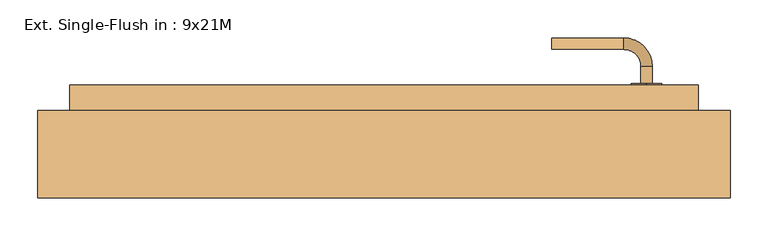
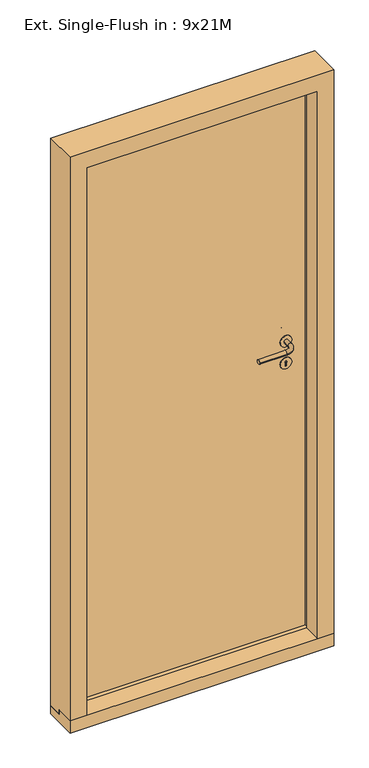
"""IFC4 building model written with IfcOpenShell, lengths in millimetres: door geometry, Ext. Single-Flush in : 9x21M."""

from ifc_helpers import new_model, si_unit, point, frame, frame_2d, origin, place, context, project, spatial, polyline, circle_curve, ellipse_curve, trimmed, segment, composite_curve, outline, extrude, faceted_brep, source, transform, mapped, element, save
from ifc_brep_helpers import plane_surface, cylinder_surface, revolved_surface, advanced_brep


def ext_single_flush_in_9x21m_f1e34a21(model_context):
    return source(origin(), model_context, "Body", "SolidModel", [
        extrude(outline(composite_curve([segment(trimmed(circle_curve(frame_2d((1090.0, 346.0)), 20.0), [point((1070.0, 346.0))], [point((1110.0, 346.0))], False, "CARTESIAN"), True, "CONTINUOUS"), segment(trimmed(circle_curve(frame_2d((1090.0, 346.0)), 20.0), [point((1110.0, 346.0))], [point((1070.0, 346.0))], False, "CARTESIAN"), True, "CONTINUOUS")], self_intersect=False)), frame((0.0, -35.0, 0.0), z_axis=(0.0, 1.0, 0.0), x_axis=(0.0, 0.0, 1.0)), (0.0, 0.0, 1.0), 2.0),
        advanced_brep(
        [(353.5, -33.0, 1090.0), (338.5, -33.0, 1090.0), (338.5, -10.5, 1090.0), (353.5, -10.5, 1090.0), (316.0, 12.0, 1090.0), (316.0, 27.0, 1090.0), (221.0, 12.0, 1090.0), (221.0, 27.0, 1090.0)],
        [
            (0, 1, circle_curve(frame((346.0, -33.0, 1090.0), z_axis=(0.0, -1.0, 0.0), x_axis=(-1.0, 0.0, 0.0)), 7.5)),
            (1, 0, circle_curve(frame((346.0, -33.0, 1090.0), z_axis=(0.0, -1.0, 0.0), x_axis=(-1.0, 0.0, 0.0)), 7.5)),
            (1, 2),
            (2, 3, circle_curve(frame((346.0, -10.5, 1090.0), z_axis=(0.0, -1.0, 0.0), x_axis=(-1.0, 0.0, 0.0)), 7.5)),
            (3, 0),
            (3, 2, circle_curve(frame((346.0, -10.5, 1090.0), z_axis=(0.0, -1.0, 0.0), x_axis=(-1.0, 0.0, 0.0)), 7.5)),
            (4, 5, circle_curve(frame((316.0, 19.5, 1090.0), z_axis=(1.0, 0.0, 0.0), x_axis=(0.0, -1.0, 0.0)), 7.5)),
            (5, 3, circle_curve(frame((316.0, -10.5, 1090.0), z_axis=(0.0, 0.0, -1.0), x_axis=(1.0, 0.0, 0.0)), 37.5)),
            (2, 4, circle_curve(frame((316.0, -10.5, 1090.0), z_axis=(0.0, 0.0, 1.0), x_axis=(1.0, 0.0, 0.0)), 22.5)),
            (5, 4, circle_curve(frame((316.0, 19.5, 1090.0), z_axis=(1.0, 0.0, 0.0), x_axis=(0.0, -1.0, 0.0)), 7.5)),
            (4, 6),
            (6, 7, circle_curve(frame((221.0, 19.5, 1090.0), z_axis=(1.0, 0.0, 0.0), x_axis=(0.0, -1.0, 0.0)), 7.5)),
            (7, 5),
            (7, 6, circle_curve(frame((221.0, 19.5, 1090.0), z_axis=(1.0, 0.0, 0.0), x_axis=(0.0, -1.0, 0.0)), 7.5)),
        ],
        [
            plane_surface(frame((346.0, -33.0, 1090.0), z_axis=(0.0, -1.0, 0.0), x_axis=(0.0, 0.0, -1.0))),
            cylinder_surface(frame((346.0, -33.0, 1090.0), z_axis=(0.0, -1.0, 0.0), x_axis=(-1.0, 0.0, 0.0)), 7.5),
            revolved_surface(trimmed(ellipse_curve(frame((346.0, -10.5, 1090.0), z_axis=(0.0, 1.0, 0.0), x_axis=(-1.0, 0.0, 0.0)), 7.5, 7.5), [point((353.5, -10.5, 1090.0))], [point((338.5, -10.5, 1090.0))], True, "CARTESIAN"), (316.0, -10.5, 1090.0), (0.0, 0.0, -1.0)),
            revolved_surface(trimmed(ellipse_curve(frame((346.0, -10.5, 1090.0), z_axis=(0.0, 1.0, 0.0), x_axis=(-1.0, 0.0, 0.0)), 7.5, 7.5), [point((338.5, -10.5, 1090.0))], [point((353.5, -10.5, 1090.0))], True, "CARTESIAN"), (316.0, -10.5, 1090.0), (0.0, 0.0, -1.0)),
            cylinder_surface(frame((316.0, 19.5, 1090.0), z_axis=(1.0, 0.0, 0.0), x_axis=(0.0, -1.0, 0.0)), 7.5),
            plane_surface(frame((221.0, 19.5, 1090.0), z_axis=(-1.0, 0.0, 0.0), x_axis=(0.0, 0.0, -1.0))),
        ],
        [
            (0, [[1, 2]]),
            (1, [[3, 4, 5, -2]]),
            (1, [[-5, 6, -3, -1]]),
            (2, [[7, 8, -4, 9]]),
            (3, [[10, -9, -6, -8]]),
            (4, [[11, 12, 13, -7]]),
            (4, [[-13, 14, -11, -10]]),
            (5, [[-12, -14]]),
        ],
    ),
        extrude(outline(composite_curve([segment(trimmed(circle_curve(frame_2d((1010.0, 346.0)), 20.0), [point((990.0, 346.0))], [point((1030.0, 346.0))], False, "CARTESIAN"), True, "CONTINUOUS"), segment(trimmed(circle_curve(frame_2d((1010.0, 346.0)), 20.0), [point((1030.0, 346.0))], [point((990.0, 346.0))], False, "CARTESIAN"), True, "CONTINUOUS")], self_intersect=False), holes=[composite_curve([segment(polyline([(1012.4019238, 347.5), (1000.0, 347.5), (1000.0, 344.5), (1012.4019238, 344.5)]), True, "CONTINUOUS"), segment(trimmed(circle_curve(frame_2d((1015.0, 346.0)), 3.0), [point((1012.4019238, 344.5))], [point((1012.4019238, 347.5))], True, "CARTESIAN"), True, "CONTINUOUS")], self_intersect=False)]), frame((0.0, -35.0, 0.0), z_axis=(0.0, 1.0, 0.0), x_axis=(0.0, 0.0, 1.0)), (0.0, 0.0, 1.0), 2.0),
        extrude(outline(composite_curve([segment(trimmed(circle_curve(frame_2d((1090.0, 346.0)), 20.0), [point((1070.0, 346.0))], [point((1110.0, 346.0))], False, "CARTESIAN"), True, "CONTINUOUS"), segment(trimmed(circle_curve(frame_2d((1090.0, 346.0)), 20.0), [point((1110.0, 346.0))], [point((1070.0, 346.0))], False, "CARTESIAN"), True, "CONTINUOUS")], self_intersect=False)), frame((0.0, -87.0, 0.0), z_axis=(0.0, 1.0, 0.0), x_axis=(0.0, 0.0, 1.0)), (0.0, 0.0, 1.0), 2.0),
        advanced_brep(
        [(353.5, -87.0, 1090.0), (338.5, -87.0, 1090.0), (353.5, -109.5, 1090.0), (338.5, -109.5, 1090.0), (316.0, -132.0, 1090.0), (316.0, -147.0, 1090.0), (221.0, -147.0, 1090.0), (221.0, -132.0, 1090.0)],
        [
            (0, 1, circle_curve(frame((346.0, -87.0, 1090.0), z_axis=(0.0, 1.0, 0.0), x_axis=(-1.0, 0.0, 0.0)), 7.5)),
            (1, 0, circle_curve(frame((346.0, -87.0, 1090.0), z_axis=(0.0, 1.0, 0.0), x_axis=(-1.0, 0.0, 0.0)), 7.5)),
            (0, 2),
            (2, 3, circle_curve(frame((346.0, -109.5, 1090.0), z_axis=(0.0, 1.0, 0.0), x_axis=(-1.0, 0.0, 0.0)), 7.5)),
            (3, 1),
            (3, 2, circle_curve(frame((346.0, -109.5, 1090.0), z_axis=(0.0, 1.0, 0.0), x_axis=(-1.0, 0.0, 0.0)), 7.5)),
            (4, 3, circle_curve(frame((316.0, -109.5, 1090.0), z_axis=(0.0, 0.0, 1.0), x_axis=(1.0, 0.0, 0.0)), 22.5)),
            (2, 5, circle_curve(frame((316.0, -109.5, 1090.0), z_axis=(0.0, 0.0, -1.0), x_axis=(1.0, 0.0, 0.0)), 37.5)),
            (5, 4, circle_curve(frame((316.0, -139.5, 1090.0), z_axis=(1.0, 0.0, 0.0), x_axis=(0.0, 1.0, 0.0)), 7.5)),
            (4, 5, circle_curve(frame((316.0, -139.5, 1090.0), z_axis=(1.0, 0.0, 0.0), x_axis=(0.0, 1.0, 0.0)), 7.5)),
            (5, 6),
            (6, 7, circle_curve(frame((221.0, -139.5, 1090.0), z_axis=(1.0, 0.0, 0.0), x_axis=(0.0, 1.0, 0.0)), 7.5)),
            (7, 4),
            (7, 6, circle_curve(frame((221.0, -139.5, 1090.0), z_axis=(1.0, 0.0, 0.0), x_axis=(0.0, 1.0, 0.0)), 7.5)),
        ],
        [
            plane_surface(frame((346.0, -87.0, 1090.0), z_axis=(0.0, 1.0, 0.0), x_axis=(0.0, 0.0, -1.0))),
            cylinder_surface(frame((346.0, -87.0, 1090.0), z_axis=(0.0, 1.0, 0.0), x_axis=(-1.0, 0.0, 0.0)), 7.5),
            revolved_surface(trimmed(ellipse_curve(frame((346.0, -109.5, 1090.0), z_axis=(0.0, 1.0, 0.0), x_axis=(-1.0, 0.0, 0.0)), 7.5, 7.5), [point((353.5, -109.5, 1090.0))], [point((338.5, -109.5, 1090.0))], True, "CARTESIAN"), (316.0, -109.5, 1090.0), (0.0, 0.0, -1.0)),
            revolved_surface(trimmed(ellipse_curve(frame((346.0, -109.5, 1090.0), z_axis=(0.0, 1.0, 0.0), x_axis=(-1.0, 0.0, 0.0)), 7.5, 7.5), [point((338.5, -109.5, 1090.0))], [point((353.5, -109.5, 1090.0))], True, "CARTESIAN"), (316.0, -109.5, 1090.0), (0.0, 0.0, -1.0)),
            cylinder_surface(frame((316.0, -139.5, 1090.0), z_axis=(1.0, 0.0, 0.0), x_axis=(0.0, 1.0, 0.0)), 7.5),
            plane_surface(frame((221.0, -139.5, 1090.0), z_axis=(-1.0, 0.0, 0.0), x_axis=(0.0, 0.0, -1.0))),
        ],
        [
            (0, [[1, 2]]),
            (1, [[-1, 3, 4, 5]]),
            (1, [[-2, -5, 6, -3]]),
            (2, [[7, -4, 8, 9]]),
            (3, [[-8, -6, -7, 10]]),
            (4, [[-9, 11, 12, 13]]),
            (4, [[-10, -13, 14, -11]]),
            (5, [[-14, -12]]),
        ],
    ),
        extrude(outline(composite_curve([segment(trimmed(circle_curve(frame_2d((1010.0, 346.0)), 20.0), [point((990.0, 346.0))], [point((1030.0, 346.0))], False, "CARTESIAN"), True, "CONTINUOUS"), segment(trimmed(circle_curve(frame_2d((1010.0, 346.0)), 20.0), [point((1030.0, 346.0))], [point((990.0, 346.0))], False, "CARTESIAN"), True, "CONTINUOUS")], self_intersect=False), holes=[composite_curve([segment(polyline([(1012.4019238, 347.5), (1000.0, 347.5), (1000.0, 344.5), (1012.4019238, 344.5)]), True, "CONTINUOUS"), segment(trimmed(circle_curve(frame_2d((1015.0, 346.0)), 3.0), [point((1012.4019238, 344.5))], [point((1012.4019238, 347.5))], True, "CARTESIAN"), True, "CONTINUOUS")], self_intersect=False)]), frame((0.0, -87.0, 0.0), z_axis=(0.0, 1.0, 0.0), x_axis=(0.0, 0.0, 1.0)), (0.0, 0.0, 1.0), 2.0),
        faceted_brep([(-414.0, -69.0, 2058.0), (-414.0, -69.0, 30.0), (-456.0, -69.0, 30.0), (-456.0, -69.0, 2100.0), (456.0, -69.0, 2100.0), (456.0, -69.0, 30.0), (414.0, -69.0, 30.0), (414.0, -69.0, 2058.0), (414.0, -119.0, 30.0), (414.0, -119.0, 45.0), (414.0, -119.0, 2058.0), (456.0, -119.0, 30.0), (-456.0, -119.0, 30.0), (-414.0, -119.0, 30.0), (456.0, -184.0, 2100.0), (456.0, -184.0, 45.0), (456.0, -119.0, 45.0), (-456.0, -119.0, 45.0), (-456.0, -184.0, 45.0), (-456.0, -184.0, 2100.0), (-414.0, -119.0, 2058.0), (-414.0, -119.0, 45.0), (-399.0, -184.0, 45.0), (-399.0, -184.0, 2043.0), (399.0, -184.0, 2043.0), (399.0, -184.0, 45.0), (399.0, -119.0, 45.0), (-399.0, -119.0, 45.0), (399.0, -119.0, 2043.0), (-399.0, -119.0, 2043.0)], [[[0, 1, 2, 3, 4, 5, 6, 7]], [[7, 6, 8, 9, 10]], [[8, 6, 5, 11]], [[12, 2, 1, 13]], [[14, 15, 16, 11, 5, 4]], [[3, 2, 12, 17, 18, 19]], [[20, 21, 13, 1, 0]], [[19, 18, 22, 23, 24, 25, 15, 14]], [[16, 15, 25, 26, 9]], [[21, 27, 22, 18, 17]], [[11, 16, 9, 8]], [[13, 21, 17, 12]], [[28, 26, 25, 24]], [[23, 22, 27, 29]], [[29, 27, 21, 20, 10, 9, 26, 28]], [[3, 19, 14, 4]], [[23, 29, 28, 24]], [[7, 10, 20, 0]]]),
        extrude(outline(polyline([(-414.0, -85.0), (-414.0, -35.0), (414.0, -35.0), (414.0, -85.0), (-414.0, -85.0)])), frame((0.0, 0.0, 30.0), z_axis=(0.0, 0.0, 1.0), x_axis=(1.0, 0.0, 0.0)), (0.0, 0.0, 1.0), 2028.0),
        extrude(outline(polyline([(-69.0, 30.0), (-69.0, 0.0), (-184.0, 0.0), (-184.0, 45.0), (-119.0, 45.0), (-119.0, 30.0), (-69.0, 30.0)])), frame((-456.0, 0.0, 0.0), z_axis=(1.0, 0.0, 0.0), x_axis=(0.0, 1.0, 0.0)), (0.0, 0.0, 1.0), 912.0),
    ])


if __name__ == "__main__":
    model = new_model("IFC4")
    model_context = context("Model", 3, world=origin())
    ifc_project = project(units=[si_unit("LENGTHUNIT", "METRE", prefix="MILLI")], contexts=[model_context])
    site = spatial("IfcSite", under=ifc_project)
    building = spatial("IfcBuilding", under=site)
    placement = place(None, origin())
    ext_single_flush_in_9x21m_shape = ext_single_flush_in_9x21m_f1e34a21(model_context)
    element("IfcDoor", 1, ObjectType="Ext. Single-Flush in : 9x21M", at=placement, inside=building, context=model_context, shape_type="MappedRepresentation", body=[
        mapped(ext_single_flush_in_9x21m_shape, transform((0.0, 0.0, 0.0), x_axis=(1.0, 0.0, 0.0), y_axis=(0.0, 1.0, 0.0), z_axis=(0.0, 0.0, 1.0))),
    ])
    save(model, "model.ifc")

# Revit data of these elements
# Type "Ext. Single-Flush in : 9x21M"
#   Type Mark = "62"
#   Sound Rating = ""
#   Opening Side [instance default] = "in"
#   Hinge Side [instance default] = ""
#   Creator Build [instance default] = "2017.0301.0"
#   Creator Organization [instance default] = "© Danish Educational Content"
#   Creator Name [instance default] = "© Erik Falck Jørgensen"
#   Analytic Construction = "<None>"
#   length#5 = 912 mm
#   length#4 = 120 mm
#   length#3 = 30 mm
#   length#2 = 57 mm
#   length#1 = 0 mm
#   Thickness = 50 mm
#   Seal Width = 12 mm
#   Rough Width = 912 mm
#   Rough Height = 2100 mm
#   Rebate Depth = 50 mm
#   Rabbet Width = 15 mm
#   Rabbet Depth = 50 mm
#   Height = 2088 mm
#   Width = 888 mm
#   Handle From Side = 110 mm
#   Handle From Bottom = 1090 mm
#   Exterior Direction [instance default] = 0.00°
#   Case Depth = 115 mm
#   Case Width = 45 mm
#   Threshold = yes
#   Sealing = no
#   Hinging = yes
#   Wall Closure = 1
#   Function = 1
#   Panel = none
#   Handle Finish = none
#   Handle = element 628255
#   Case/Transom = none
#   Assembly Code = ""
# Element 1 (IfcDoor, "Ext. Single-Flush in : 9x21M")
#   Materials on its faces: "Stainless Steel, Polished", "Default Frame/Mullion (Interior/Exterior)", "Default Door Panel (Exterior/Interior)"
# Materials
#   "Stainless Steel, Polished": class "Metal", colour RGB 180 180 180, transparency 0, Description = "Rustfri stål, poleret", Cost = 0
#   "Default Frame/Mullion (Interior/Exterior)": class "Generic", colour RGB 205 205 205, transparency 0, Description = "Udefineret karm/ramme materiale", Cost = 0
#   "Default Door Panel (Exterior/Interior)": class "Generic", colour RGB 205 205 205, transparency 0, Description = "Udefineret dørplade materiale", Cost = 0
